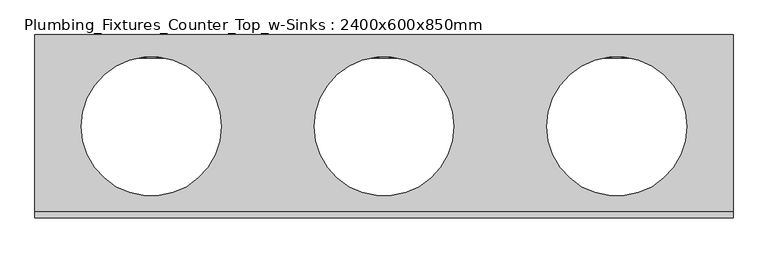
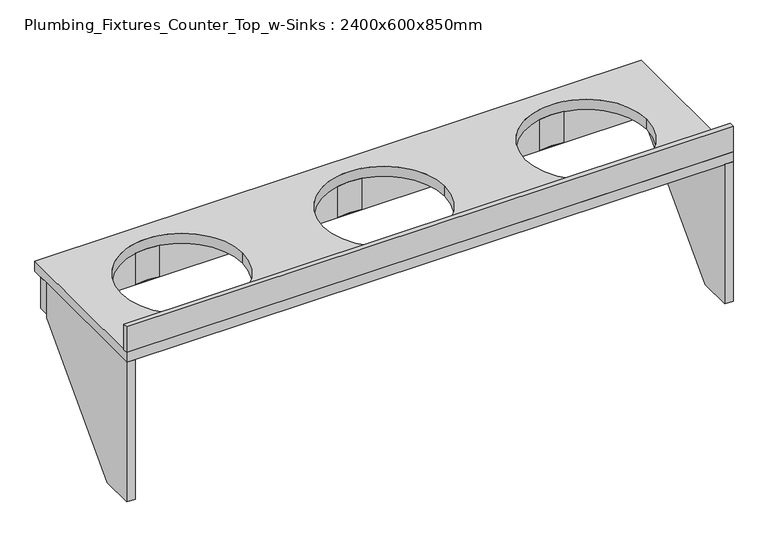
"""IFC4 building model written with IfcOpenShell, lengths in millimetres: furniture geometry, Plumbing_Fixtures_Counter_Top_w-Sinks : 2400x600x850mm."""

from ifc_helpers import new_model, si_unit, point, frame, frame_2d, origin, place, context, project, spatial, polyline, circle_curve, trimmed, segment, composite_curve, outline, extrude, source, transform, mapped, element, save
from ifc_brep_helpers import plane_surface, revolved_surface, advanced_brep


def plumbing_fixtures_counter_top_w_sinks_2400x600x850mm_820859b4(model_context):
    return source(origin(), model_context, "Body", "SolidModel", [
        extrude(outline(polyline([(69.85, 810.0), (593.65, 810.0), (593.65, 670.3), (196.85, 254.0), (69.85, 254.0), (69.85, 810.0)])), frame((-1116.1103038, 0.0, 0.0), z_axis=(1.0, 0.0, 0.0), x_axis=(0.0, 1.0, 0.0)), (0.0, 0.0, 1.0), 31.75),
        extrude(outline(polyline([(69.85, 810.0), (593.65, 810.0), (593.65, 670.3), (196.85, 254.0), (69.85, 254.0), (69.85, 810.0)])), frame((1138.1396962, 0.0, 0.0), z_axis=(1.0, 0.0, 0.0), x_axis=(0.0, 1.0, 0.0)), (0.0, 0.0, 1.0), 31.75),
        advanced_brep(
        [(-1116.1103038, 593.65, 810.0), (-1116.1103038, 631.75, 810.0), (-1116.1103038, 631.75, 685.0), (-1116.1103038, 593.65, 685.0), (1169.8896962, 593.65, 810.0), (1169.8896962, 593.65, 685.0), (1169.8896962, 631.75, 685.0), (1169.8896962, 631.75, 810.0), (-781.7098746, 593.65, 810.0), (-688.510733, 593.65, 810.0), (-19.7098746, 593.65, 810.0), (73.489267, 593.65, 810.0), (742.2901254, 593.65, 810.0), (835.489267, 593.65, 810.0), (835.489267, 593.65, 686.2), (742.2901254, 593.65, 686.2), (73.489267, 593.65, 685.8), (-19.7098746, 593.65, 685.8), (-688.510733, 593.65, 685.4), (-781.7098746, 593.65, 685.4)],
        [
            (0, 1),
            (1, 2),
            (2, 3),
            (3, 0),
            (4, 5),
            (5, 6),
            (6, 7),
            (7, 4),
            (0, 8),
            (8, 9, circle_curve(frame((-735.1103038, 369.85, 810.0), z_axis=(0.0, 0.0, -1.0), x_axis=(1.0, 0.0, 0.0)), 228.6)),
            (9, 10),
            (10, 11, circle_curve(frame((26.8896962, 369.85, 810.0), z_axis=(0.0, 0.0, -1.0), x_axis=(1.0, 0.0, 0.0)), 228.6)),
            (11, 12),
            (12, 13, circle_curve(frame((788.8896962, 369.85, 810.0), z_axis=(0.0, 0.0, -1.0), x_axis=(1.0, 0.0, 0.0)), 228.6)),
            (13, 4),
            (7, 1),
            (6, 2),
            (5, 3),
            (13, 14),
            (14, 15),
            (15, 12),
            (11, 16),
            (16, 17),
            (17, 10),
            (9, 18),
            (18, 19),
            (19, 8),
            (18, 19, circle_curve(frame((-735.1103038, 369.85, 685.4), z_axis=(0.0, 0.0, 1.0), x_axis=(1.0, 0.0, 0.0)), 228.6)),
            (14, 15, circle_curve(frame((788.8896962, 369.85, 686.2), z_axis=(0.0, 0.0, 1.0), x_axis=(1.0, 0.0, 0.0)), 228.6)),
            (16, 17, circle_curve(frame((26.8896962, 369.85, 685.8), z_axis=(0.0, 0.0, 1.0), x_axis=(1.0, 0.0, 0.0)), 228.6)),
        ],
        [
            plane_surface(frame((-1116.1103038, 631.75, 810.0), z_axis=(-1.0, 0.0, 0.0), x_axis=(0.0, 1.0, 0.0))),
            plane_surface(frame((1169.8896962, 631.75, 810.0), z_axis=(1.0, 0.0, 0.0), x_axis=(0.0, -1.0, 0.0))),
            plane_surface(frame((-1116.1103038, 593.65, 810.0), z_axis=(0.0, 0.0, 1.0), x_axis=(1.0, 0.0, 0.0))),
            plane_surface(frame((-1116.1103038, 631.75, 810.0), z_axis=(0.0, 1.0, 0.0), x_axis=(1.0, 0.0, 0.0))),
            plane_surface(frame((-1116.1103038, 631.75, 685.0), z_axis=(0.0, 0.0, -1.0), x_axis=(1.0, 0.0, 0.0))),
            plane_surface(frame((-1116.1103038, 593.65, 685.0), z_axis=(0.0, -1.0, 0.0), x_axis=(1.0, 0.0, 0.0))),
            plane_surface(frame((-506.5103038, 369.85, 685.4), z_axis=(0.0, 0.0, 1.0), x_axis=(0.0, -1.0, 0.0))),
            revolved_surface(polyline([(-506.5103038, 369.85, 810.0), (-506.5103038, 369.85, 685.4)]), (-735.1103038, 369.85, 685.4), (0.0, 0.0, 1.0)),
            plane_surface(frame((1017.4896962, 369.85, 686.2), z_axis=(0.0, 0.0, 1.0), x_axis=(0.0, -1.0, 0.0))),
            revolved_surface(polyline([(1017.4896962, 369.85, 810.0), (1017.4896962, 369.85, 686.2)]), (788.8896962, 369.85, 686.2), (0.0, 0.0, 1.0)),
            plane_surface(frame((255.4896962, 369.85, 685.8), z_axis=(0.0, 0.0, 1.0), x_axis=(0.0, -1.0, 0.0))),
            revolved_surface(polyline([(255.4896962, 369.85, 810.0), (255.4896962, 369.85, 685.8)]), (26.8896962, 369.85, 685.8), (0.0, 0.0, 1.0)),
        ],
        [
            (0, [[1, 2, 3, 4]]),
            (1, [[5, 6, 7, 8]]),
            (2, [[-1, 9, 10, 11, 12, 13, 14, 15, -8, 16]]),
            (3, [[-2, -16, -7, 17]]),
            (4, [[-3, -17, -6, 18]]),
            (5, [[-4, -18, -5, -15, 19, 20, 21, -13, 22, 23, 24, -11, 25, 26, 27, -9]]),
            (6, [[28, -26]]),
            (7, [[-28, -25, -10, -27]]),
            (8, [[29, -20]]),
            (9, [[-29, -19, -14, -21]]),
            (10, [[30, -23]]),
            (11, [[-30, -22, -12, -24]]),
        ],
    ),
        extrude(outline(polyline([(1169.8896962, 69.85), (-1116.1103038, 69.85), (-1116.1103038, 88.9), (1169.8896962, 88.9), (1169.8896962, 69.85)])), frame((0.0, 0.0, 850.0), z_axis=(0.0, 0.0, 1.0), x_axis=(1.0, 0.0, 0.0)), (0.0, 0.0, 1.0), 101.6),
        extrude(outline(polyline([(1169.8896962, 69.85), (-1116.1103038, 69.85), (-1116.1103038, 669.85), (1169.8896962, 669.85), (1169.8896962, 69.85)]), holes=[composite_curve([segment(trimmed(circle_curve(frame_2d((-735.1103038, 369.85)), 228.6), [point((-963.7103038, 369.85))], [point((-506.5103038, 369.85))], True, "CARTESIAN"), True, "CONTINUOUS"), segment(trimmed(circle_curve(frame_2d((-735.1103038, 369.85)), 228.6), [point((-506.5103038, 369.85))], [point((-963.7103038, 369.85))], True, "CARTESIAN"), True, "CONTINUOUS")], self_intersect=False), composite_curve([segment(trimmed(circle_curve(frame_2d((788.8896962, 369.85)), 228.6), [point((560.2896962, 369.85))], [point((1017.4896962, 369.85))], True, "CARTESIAN"), True, "CONTINUOUS"), segment(trimmed(circle_curve(frame_2d((788.8896962, 369.85)), 228.6), [point((1017.4896962, 369.85))], [point((560.2896962, 369.85))], True, "CARTESIAN"), True, "CONTINUOUS")], self_intersect=False), composite_curve([segment(trimmed(circle_curve(frame_2d((26.8896962, 369.85)), 228.6), [point((-201.7103038, 369.85))], [point((255.4896962, 369.85))], True, "CARTESIAN"), True, "CONTINUOUS"), segment(trimmed(circle_curve(frame_2d((26.8896962, 369.85)), 228.6), [point((255.4896962, 369.85))], [point((-201.7103038, 369.85))], True, "CARTESIAN"), True, "CONTINUOUS")], self_intersect=False)]), frame((0.0, 0.0, 810.0), z_axis=(0.0, 0.0, 1.0), x_axis=(1.0, 0.0, 0.0)), (0.0, 0.0, 1.0), 40.0),
    ])


if __name__ == "__main__":
    model = new_model("IFC4")
    model_context = context("Model", 3, world=origin())
    ifc_project = project(units=[si_unit("LENGTHUNIT", "METRE", prefix="MILLI")], contexts=[model_context])
    site = spatial("IfcSite", under=ifc_project)
    building = spatial("IfcBuilding", under=site)
    placement = place(None, origin())
    plumbing_fixtures_counter_top_w_sinks_2400x600x850mm_shape = plumbing_fixtures_counter_top_w_sinks_2400x600x850mm_820859b4(model_context)
    element("IfcFurniture", 1, ObjectType="Plumbing_Fixtures_Counter_Top_w-Sinks : 2400x600x850mm", at=placement, inside=building, context=model_context, shape_type="MappedRepresentation", body=[
        mapped(plumbing_fixtures_counter_top_w_sinks_2400x600x850mm_shape, transform((0.0, 0.0, 0.0), x_axis=(1.0, 0.0, 0.0), y_axis=(0.0, 1.0, 0.0), z_axis=(0.0, 0.0, 1.0))),
    ])
    save(model, "model.ifc")

# Revit data of these elements
# Type "Plumbing_Fixtures_Counter_Top_w-Sinks : 2400x600x850mm"
#   Keynote = "N13/180"
#   Assembly Code = "C1030400"
#   Height = 2' - 9.46457"
#   Distance To Sink Center [instance default] = 1' - 3"
#   Clear Space = 2' - 2.9685"
#   Counter Thickness = 0' - 1.5748"
#   Depth = 1' - 11.62205"
#   Length [instance default] = 7' - 6"
#   Number Of Sinks [instance default] = 3
#   Counter Top Material = Laminate
#   Base Material = Laminate
#   Default Elevation = 0
# Element 1 (IfcFurniture, "Plumbing_Fixtures_Counter_Top_w-Sinks : 2400x600x850mm")
#   Materials on its faces: "Laminate"
# Materials
#   "Laminate": class "Miscellaneous", colour RGB 247 235 201, transparency 0
